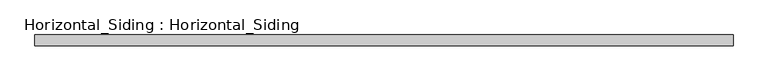
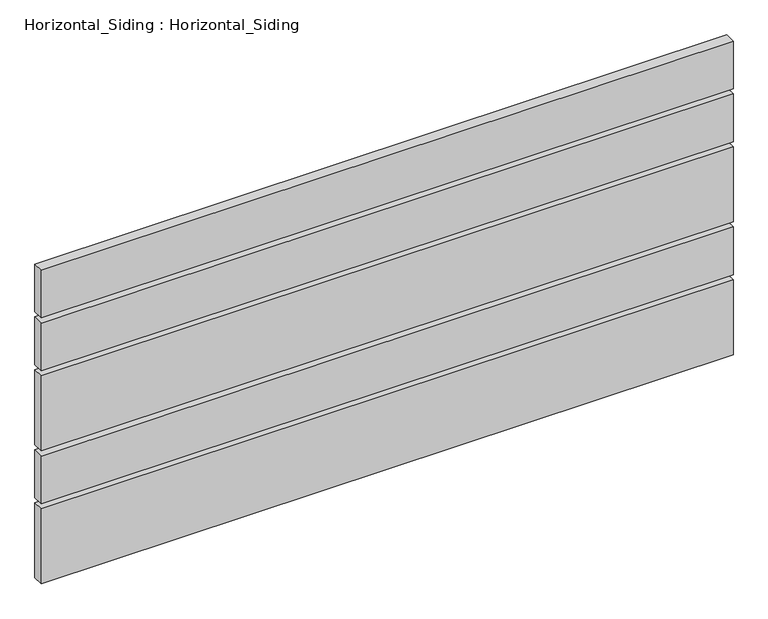
"""IFC4 building model written with IfcOpenShell, lengths in millimetres: plate geometry, Horizontal_Siding : Horizontal_Siding."""

from ifc_helpers import new_model, si_unit, frame, origin, place, context, project, spatial, polyline, outline, extrude, source, transform, mapped, element, save


def horizontal_siding_horizontal_siding_07e4e943(model_context):
    return source(origin(), model_context, "Body", "SweptSolid", [
        extrude(outline(polyline([(609.6, -19.05), (-609.6, -19.05), (-609.6, 0.0), (609.6, 0.0), (609.6, -19.05)])), frame((0.0, 0.0, 9.525), z_axis=(0.0, 0.0, 1.0), x_axis=(1.0, 0.0, 0.0)), (0.0, 0.0, 1.0), 139.7),
        extrude(outline(polyline([(609.6, -19.05), (-609.6, -19.05), (-609.6, 0.0), (609.6, 0.0), (609.6, -19.05)])), frame((0.0, 0.0, 158.75), z_axis=(0.0, 0.0, 1.0), x_axis=(1.0, 0.0, 0.0)), (0.0, 0.0, 1.0), 88.9),
        extrude(outline(polyline([(609.6, -19.05), (-609.6, -19.05), (-609.6, 0.0), (609.6, 0.0), (609.6, -19.05)])), frame((0.0, 0.0, 257.175), z_axis=(0.0, 0.0, 1.0), x_axis=(1.0, 0.0, 0.0)), (0.0, 0.0, 1.0), 139.7),
        extrude(outline(polyline([(609.6, -19.05), (-609.6, -19.05), (-609.6, 0.0), (609.6, 0.0), (609.6, -19.05)])), frame((0.0, 0.0, 406.4), z_axis=(0.0, 0.0, 1.0), x_axis=(1.0, 0.0, 0.0)), (0.0, 0.0, 1.0), 88.9),
        extrude(outline(polyline([(609.6, -19.05), (-609.6, -19.05), (-609.6, 0.0), (609.6, 0.0), (609.6, -19.05)])), frame((0.0, 0.0, 504.825), z_axis=(0.0, 0.0, 1.0), x_axis=(1.0, 0.0, 0.0)), (0.0, 0.0, 1.0), 88.9),
    ])


if __name__ == "__main__":
    model = new_model("IFC4")
    model_context = context("Model", 3, world=origin())
    ifc_project = project(units=[si_unit("LENGTHUNIT", "METRE", prefix="MILLI")], contexts=[model_context])
    site = spatial("IfcSite", under=ifc_project)
    building = spatial("IfcBuilding", under=site)
    placement = place(None, origin())
    horizontal_siding_horizontal_siding_shape = horizontal_siding_horizontal_siding_07e4e943(model_context)
    element("IfcPlate", 1, ObjectType="Horizontal_Siding : Horizontal_Siding", at=placement, inside=building, context=model_context, shape_type="MappedRepresentation", body=[
        mapped(horizontal_siding_horizontal_siding_shape, transform((0.0, 0.0, 0.0), x_axis=(1.0, 0.0, 0.0), y_axis=(0.0, 1.0, 0.0), z_axis=(0.0, 0.0, 1.0))),
    ])
    save(model, "model.ifc")

# Revit data of these elements
# Type "Horizontal_Siding : Horizontal_Siding"
#   Type Mark = "OUT"
#   Analytic Construction = "<None>"
#   extend = 0' - 2 3/4"
#   Width_2 = 0' - 3 1/2"
#   Width_1 = 0' - 5 1/2"
#   Gap = 0' - 0 3/8"
#   Plank Material = EXISTING HORZ. (1X4 & 1X6) WOOD SIDING (UNGROOVED PROFILE)
# Element 1 (IfcPlate, "Horizontal_Siding : Horizontal_Siding")
#   Materials on its faces: "EXISTING HORZ. (1X4 & 1X6) WOOD SIDING (UNGROOVED PROFILE)"
# Materials
#   "EXISTING HORZ. (1X4 & 1X6) WOOD SIDING (UNGROOVED PROFILE)": class "Wood", colour RGB 164 134 123, transparency 0, Description = "Pinus Echinata", Cost = 0
